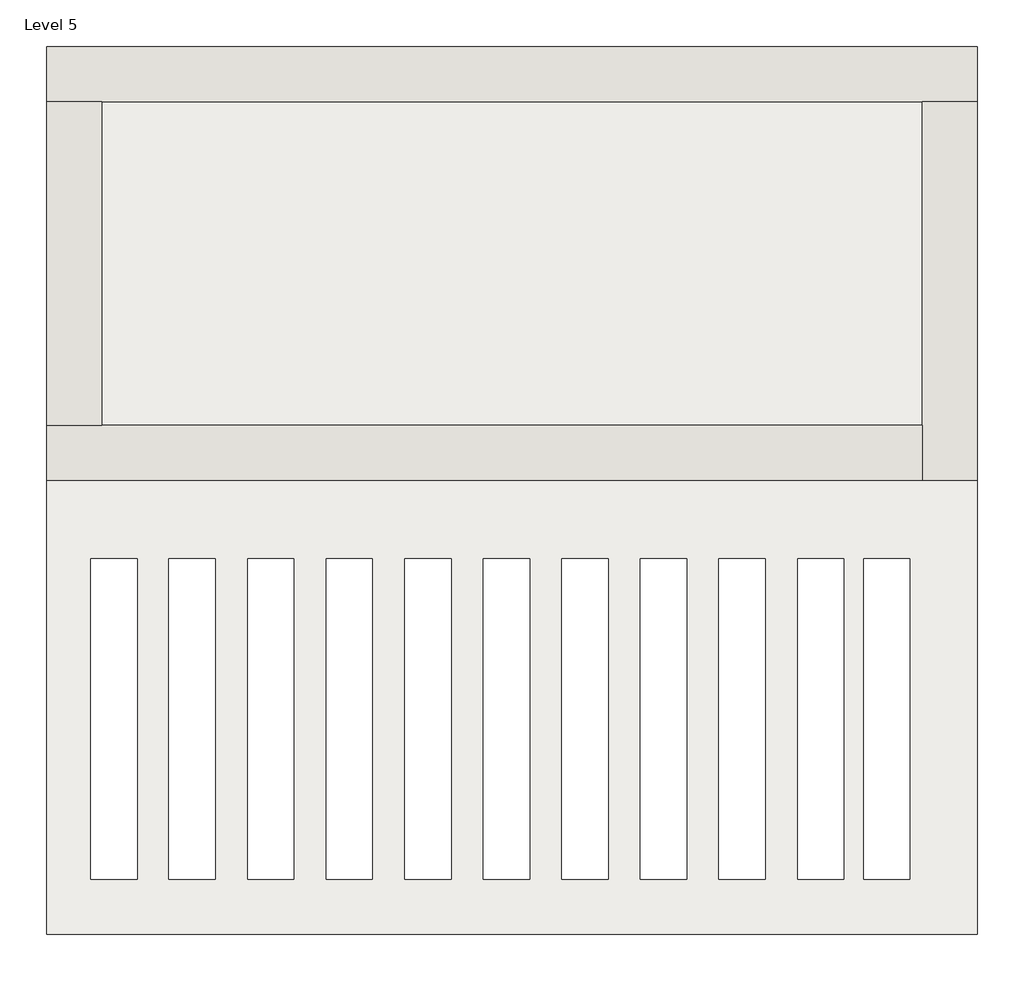
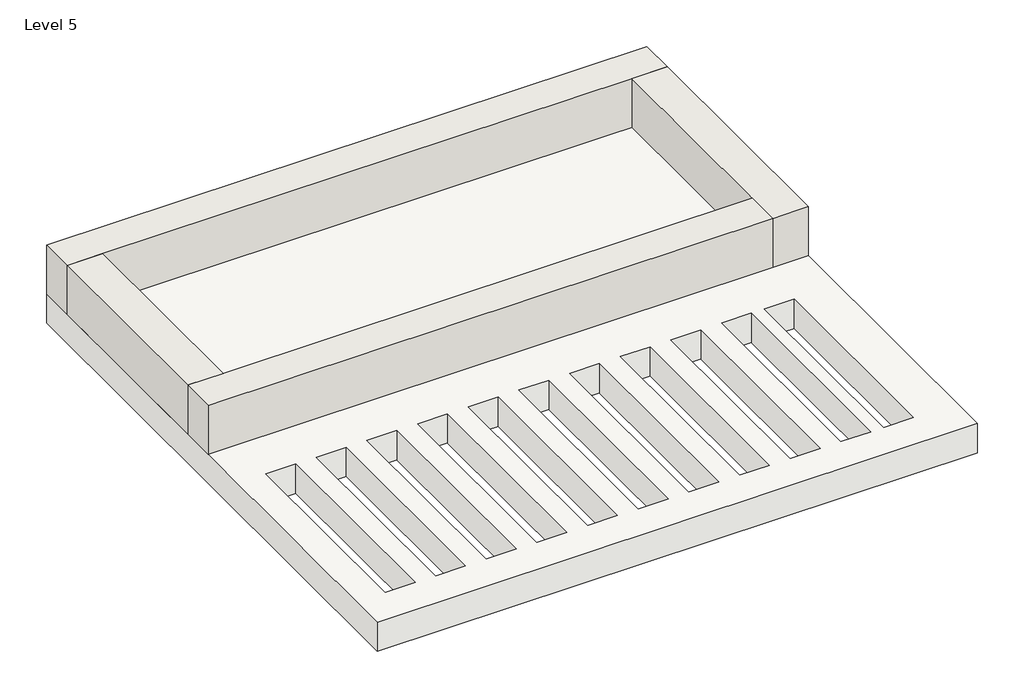
# One storey: 4 walls, 1 slab.
"""IFC4 building model written with IfcOpenShell, lengths in millimetres."""

from ifc_helpers import new_model, si_unit, frame, origin, place, context, project, spatial, polyline, outline, extrude, faceted_brep, element, save

model = new_model("IFC4")

# Units and contexts
model_context = context("Model", 3, world=origin())
ifc_project = project(units=[si_unit("LENGTHUNIT", "METRE", prefix="MILLI")], contexts=[model_context])

# Site, building, storey
site = spatial("IfcSite", under=ifc_project)
building = spatial("IfcBuilding", under=site)
storey = spatial("IfcBuildingStorey", under=building, Name="Level 5", Elevation=7925.0)

# Slab
placement = place(None, origin())
element("IfcSlab", 1, ObjectType="Generic - 12\" 2", at=placement, inside=storey, context=model_context, shape_type="SweptSolid", body=[
    extrude(outline(polyline([(-10714.2211091, -829.1492854), (-10714.2211091, 4820.8507146), (-4790.2211091, 4820.8507146), (-4790.2211091, -829.1492854), (-10714.2211091, -829.1492854)]), holes=[polyline([(-5515.2211091, 1560.8507146), (-5515.2211091, -479.1492854), (-5220.2211091, -479.1492854), (-5220.2211091, 1560.8507146), (-5515.2211091, 1560.8507146)]), polyline([(-5935.2211091, 1560.8507146), (-5935.2211091, -479.1492854), (-5640.2211091, -479.1492854), (-5640.2211091, 1560.8507146), (-5935.2211091, 1560.8507146)]), polyline([(-6435.2211091, 1560.8507146), (-6435.2211091, -479.1492854), (-6140.2211091, -479.1492854), (-6140.2211091, 1560.8507146), (-6435.2211091, 1560.8507146)]), polyline([(-6935.2211091, 1560.8507146), (-6935.2211091, -479.1492854), (-6640.2211091, -479.1492854), (-6640.2211091, 1560.8507146), (-6935.2211091, 1560.8507146)]), polyline([(-7435.2211091, 1560.8507146), (-7435.2211091, -479.1492854), (-7140.2211091, -479.1492854), (-7140.2211091, 1560.8507146), (-7435.2211091, 1560.8507146)]), polyline([(-7935.2211091, 1560.8507146), (-7935.2211091, -479.1492854), (-7640.2211091, -479.1492854), (-7640.2211091, 1560.8507146), (-7935.2211091, 1560.8507146)]), polyline([(-8435.2211091, 1560.8507146), (-8435.2211091, -479.1492854), (-8140.2211091, -479.1492854), (-8140.2211091, 1560.8507146), (-8435.2211091, 1560.8507146)]), polyline([(-8935.2211091, 1560.8507146), (-8935.2211091, -479.1492854), (-8640.2211091, -479.1492854), (-8640.2211091, 1560.8507146), (-8935.2211091, 1560.8507146)]), polyline([(-9435.2211091, 1560.8507146), (-9435.2211091, -479.1492854), (-9140.2211091, -479.1492854), (-9140.2211091, 1560.8507146), (-9435.2211091, 1560.8507146)]), polyline([(-9935.2211091, 1560.8507146), (-9935.2211091, -479.1492854), (-9640.2211091, -479.1492854), (-9640.2211091, 1560.8507146), (-9935.2211091, 1560.8507146)]), polyline([(-10432.899203, 1560.8507146), (-10432.899203, -479.1492854), (-10137.899203, -479.1492854), (-10137.899203, 1560.8507146), (-10432.899203, 1560.8507146)])]), frame((0.0, 0.0, 7925.0), z_axis=(0.0, 0.0, 1.0), x_axis=(1.0, 0.0, 0.0)), (0.0, 0.0, 1.0), 304.8),
])

# Walls
element("IfcWall", 2, ObjectType="wall 351", at=placement, inside=storey, context=model_context, shape_type="Brep", body=[
    faceted_brep([(-10714.2211091, 4470.8507146, 8229.8), (-10364.2211091, 4470.8507146, 8229.8), (-5140.2211091, 4470.8507146, 8229.8), (-4790.2211091, 4470.8507146, 8229.8), (-4790.2211091, 4470.8507146, 8739.9228942), (-5140.2211091, 4470.8507146, 8739.9228942), (-10364.2211091, 4470.8507146, 8739.9228942), (-10714.2211091, 4470.8507146, 8739.9228942), (-10714.2211091, 4820.8507146, 8229.8), (-10714.2211091, 4820.8507146, 8739.9228942), (-4790.2211091, 4820.8507146, 8739.9228942), (-4790.2211091, 4820.8507146, 8229.8)], [[[0, 1, 2, 3, 4, 5, 6, 7]], [[8, 9, 10, 11]], [[3, 2, 1, 0, 8, 11]], [[7, 6, 5, 4, 10, 9]], [[4, 3, 11, 10]], [[0, 7, 9, 8]]]),
])
element("IfcWall", 3, ObjectType="wall 351", at=placement, inside=storey, context=model_context, shape_type="Brep", body=[
    faceted_brep([(-5140.2211091, 4470.8507146, 8229.8), (-5140.2211091, 2410.8507146, 8229.8), (-5140.2211091, 2060.8507146, 8229.8), (-5140.2211091, 2060.8507146, 8739.9228942), (-5140.2211091, 2410.8507146, 8739.9228942), (-5140.2211091, 4470.8507146, 8739.9228942), (-4790.2211091, 4470.8507146, 8229.8), (-4790.2211091, 4470.8507146, 8739.9228942), (-4790.2211091, 2060.8507146, 8739.9228942), (-4790.2211091, 2060.8507146, 8229.8)], [[[0, 1, 2, 3, 4, 5]], [[6, 7, 8, 9]], [[2, 1, 0, 6, 9]], [[5, 4, 3, 8, 7]], [[0, 5, 7, 6]], [[3, 2, 9, 8]]]),
])
element("IfcWall", 4, ObjectType="wall 351", at=placement, inside=storey, context=model_context, shape_type="Brep", body=[
    faceted_brep([(-5140.2211091, 2410.8507146, 8229.8), (-10364.2211091, 2410.8507146, 8229.8), (-10714.2211091, 2410.8507146, 8229.8), (-10714.2211091, 2410.8507146, 8739.9228942), (-10364.2211091, 2410.8507146, 8739.9228942), (-5140.2211091, 2410.8507146, 8739.9228942), (-5140.2211091, 2060.8507146, 8229.8), (-5140.2211091, 2060.8507146, 8739.9228942), (-10714.2211091, 2060.8507146, 8739.9228942), (-10714.2211091, 2060.8507146, 8229.8)], [[[0, 1, 2, 3, 4, 5]], [[6, 7, 8, 9]], [[2, 1, 0, 6, 9]], [[5, 4, 3, 8, 7]], [[3, 2, 9, 8]], [[0, 5, 7, 6]]]),
])
element("IfcWall", 5, ObjectType="wall 351", at=placement, inside=storey, context=model_context, shape_type="SweptSolid", body=[
    extrude(outline(polyline([(-10364.2211091, 4470.8507146), (-10364.2211091, 2410.8507146), (-10714.2211091, 2410.8507146), (-10714.2211091, 4470.8507146), (-10364.2211091, 4470.8507146)])), frame((0.0, 0.0, 8229.8), z_axis=(0.0, 0.0, 1.0), x_axis=(1.0, 0.0, 0.0)), (0.0, 0.0, 1.0), 510.1228942),
])

save(model, "model.ifc")

# Revit data of these elements
# Project information
#   项目发布日期 = "Issue Date"
#   项目状态 = "Project Status"
#   客户姓名 = "Owner"
#   项目地址 = "Enter address here"
#   项目名称 = "Project Name"
#   项目编号 = "Project Number"
# Type "Generic - 12\" 2"
#   Assembly Code = "B1010"
#   Thickness = 304.8 mm
#   Function = 0
#   Layers, outside or top first: 304.8 mm "Acoustic Ceiling Tile 24\" x 24\" 2" (function 1)
# Type "wall 351"
#   Assembly Code = "B2010"
#   Width = 350 mm
#   Layers, outside or top first: 350 mm "wall 9\" 3" (function 1)
# Element 1 (IfcSlab, "Generic - 12\" 2")
#   built-in parameter 1001955 = 3.14159 (stored number, unit not read)
#   Height Offset From Level = 304.8 mm
#   Phase Created = New Construction
#   Materials on its faces: "Acoustic Ceiling Tile 24\" x 24\" 2"
# Elements 2, 3, 4, 5 (IfcWall, "wall 351")
#   built-in parameter 1001111 = 304.8 mm
#   Top Offset = 205.923 mm
#   Base Offset = 304.8 mm
#   wall height = 510.123 mm
#   Phase Created = New Construction
#   Base Constraint = Level 5
#   Top Constraint = Level 6
#   Materials on its faces: "wall 9\" 3"
# Materials
#   "Acoustic Ceiling Tile 24\" x 24\" 2": class "Miscellaneous", colour RGB 66 30 10, transparency 0, Description = "Interior finish"
#   "wall 9\" 3": class "Miscellaneous", colour RGB 242 242 255, transparency 0, Description = "Interior finish"
